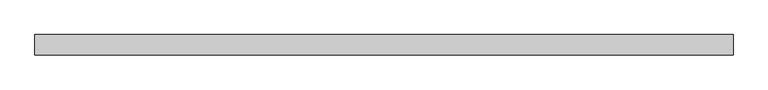
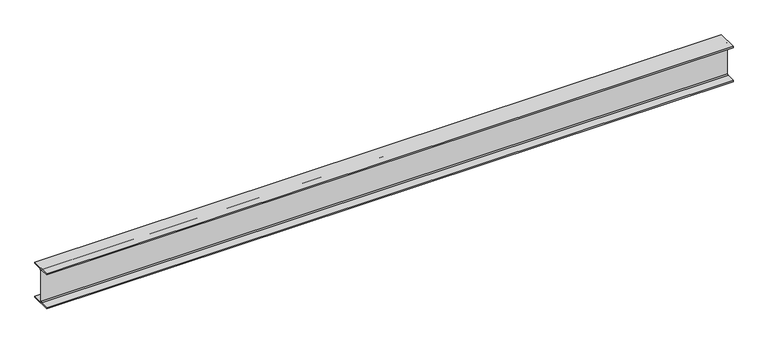
"""IFC4 building model written with IfcOpenShell, lengths in millimetres: beam geometry, Old_Steel Beam_H-KSD3502 : H_SB_ASB_H-200×200x8x12."""

import ifcopenshell
import ifcopenshell.guid

model = None  # the IFC model being written
_history = None  # IfcOwnerHistory: only IFC2X3 demands one
_inside = {}  # id of a spatial element -> (the spatial element, [elements in it])
_under = {}  # id of a project, library or spatial element -> (it, [spatial elements below it])
_declared = {}  # id of a project -> (the project, [libraries it declares])
_typed = {}  # id of a type object -> (the type object, [elements of that type])
_made_of = {}  # id of a material, layer set ... -> (it, [elements and type objects made of it])


def new_model(schema):
    """Start an empty IFC model of exactly this schema.

    Asked for "IFC4X3", IfcOpenShell would pick the latest addendum, in which some entities
    have other attributes; the version numbers below select the first issue.
    IFC2X3 requires an IfcOwnerHistory on every rooted entity: one is made here for all.
    """
    global model, _history
    if schema == "IFC4X3":
        model = ifcopenshell.file(schema_version=(4, 3, 0, 0))
    else:
        model = ifcopenshell.file(schema=schema)
    _inside.clear()
    _under.clear()
    _declared.clear()
    _typed.clear()
    _made_of.clear()
    _history = None
    if model.schema == "IFC2X3":
        org = make("IfcOrganization", Name="unknown")
        user = make(
            "IfcPersonAndOrganization",
            ThePerson=make("IfcPerson", FamilyName="unknown"),
            TheOrganization=org,
        )
        app = make(
            "IfcApplication",
            ApplicationDeveloper=org,
            Version="unknown",
            ApplicationFullName="unknown",
            ApplicationIdentifier="unknown",
        )
        _history = make(
            "IfcOwnerHistory",
            OwningUser=user,
            OwningApplication=app,
            ChangeAction="ADDED",
            CreationDate=0,
        )
    return model


def make(cls, **values):
    """One entity of the class cls with the attributes given. An attribute that is None is left unset."""
    return model.create_entity(
        cls, **{name: value for name, value in values.items() if value is not None}
    )


def rooted(cls, **values):
    """An entity with a GlobalId (a new one), such as an element, a storey or a relation."""
    return make(cls, GlobalId=ifcopenshell.guid.new(), OwnerHistory=_history, **values)


def si_unit(unit_type, name, prefix=None):
    """IfcSIUnit, for example si_unit("LENGTHUNIT", "METRE", prefix="MILLI")."""
    return make("IfcSIUnit", UnitType=unit_type, Prefix=prefix, Name=name)


def assignment(units):
    """IfcUnitAssignment: the units of a project."""
    return None if units is None else make("IfcUnitAssignment", Units=units)


def point(xyz):
    """IfcCartesianPoint."""
    return None if xyz is None else make("IfcCartesianPoint", Coordinates=xyz)


def direction(xyz):
    """IfcDirection."""
    return None if xyz is None else make("IfcDirection", DirectionRatios=xyz)


def frame(location, z_axis=None, x_axis=None):
    """IfcAxis2Placement3D, a coordinate frame: its origin and axes. An axis left out is left unset."""
    return make(
        "IfcAxis2Placement3D",
        Location=point(location),
        Axis=direction(z_axis),
        RefDirection=direction(x_axis),
    )


def frame_2d(location, x_axis=None):
    """IfcAxis2Placement2D, a coordinate frame in the plane: its origin and x axis."""
    return make(
        "IfcAxis2Placement2D", Location=point(location), RefDirection=direction(x_axis)
    )


def origin():
    """The frame at (0, 0, 0) with its axes left unset."""
    return frame((0.0, 0.0, 0.0))


def place(relative_to, where):
    """IfcLocalPlacement: puts the frame where relative to a parent placement (None: the world)."""
    return make(
        "IfcLocalPlacement", PlacementRelTo=relative_to, RelativePlacement=where
    )


def context(
    kind, dimensions, precision=None, world=None, true_north=None, identifier=None
):
    """IfcGeometricRepresentationContext, for example the 3D "Model" context."""
    return make(
        "IfcGeometricRepresentationContext",
        ContextIdentifier=identifier,
        ContextType=kind,
        CoordinateSpaceDimension=dimensions,
        Precision=precision,
        WorldCoordinateSystem=world,
        TrueNorth=true_north,
    )


def project(units=None, contexts=None):
    """IfcProject with its units and contexts."""
    return rooted(
        "IfcProject",
        Name="project",
        RepresentationContexts=contexts,
        UnitsInContext=assignment(units),
    )


def spatial(cls, under=None, at=None, **own):
    """A site, building, storey or space (cls), placed at a placement, below another one or the project."""
    s = rooted(cls, ObjectPlacement=at, **own)
    if under is not None:
        _under.setdefault(under.id(), (under, []))[1].append(s)
    return s


def polyline(points):
    """IfcPolyline through the points."""
    return make("IfcPolyline", Points=[point(p) for p in points])


def circle_curve(where, radius):
    """IfcCircle in the frame where."""
    return make("IfcCircle", Position=where, Radius=radius)


def trimmed(basis, trim1, trim2, sense, master):
    """IfcTrimmedCurve: the piece of a basis curve between two trims."""
    return make(
        "IfcTrimmedCurve",
        BasisCurve=basis,
        Trim1=trim1,
        Trim2=trim2,
        SenseAgreement=sense,
        MasterRepresentation=master,
    )


def segment(curve, same_sense, transition):
    """IfcCompositeCurveSegment."""
    return make(
        "IfcCompositeCurveSegment",
        Transition=transition,
        SameSense=same_sense,
        ParentCurve=curve,
    )


def composite_curve(segments, self_intersect=None):
    """IfcCompositeCurve: segments joined end to end."""
    return make("IfcCompositeCurve", Segments=segments, SelfIntersect=self_intersect)


def outline(outer, holes=None, kind="AREA"):
    """IfcArbitraryClosedProfileDef: a profile drawn as a closed curve; with holes, ...WithVoids."""
    if holes is None:
        return make("IfcArbitraryClosedProfileDef", ProfileType=kind, OuterCurve=outer)
    return make(
        "IfcArbitraryProfileDefWithVoids",
        ProfileType=kind,
        OuterCurve=outer,
        InnerCurves=holes,
    )


def extrude(swept, where, along, depth):
    """IfcExtrudedAreaSolid: the profile swept, set in the frame where, extruded along a direction by depth."""
    return make(
        "IfcExtrudedAreaSolid",
        SweptArea=swept,
        Position=where,
        ExtrudedDirection=direction(along),
        Depth=depth,
    )


def shape(context_of_items, identifier, shape_type, items):
    """IfcShapeRepresentation: the items that make up one representation, for example the "Body"."""
    return make(
        "IfcShapeRepresentation",
        ContextOfItems=context_of_items,
        RepresentationIdentifier=identifier,
        RepresentationType=shape_type,
        Items=items,
    )


def source(mapping_origin, context_of_items, identifier, shape_type, items):
    """IfcRepresentationMap: a shape defined once, which mapped items show again and again."""
    return make(
        "IfcRepresentationMap",
        MappingOrigin=mapping_origin,
        MappedRepresentation=shape(context_of_items, identifier, shape_type, items),
    )


def transform(
    local_origin,
    x_axis=None,
    y_axis=None,
    z_axis=None,
    scale=None,
    scale2=None,
    scale3=None,
    uniform=True,
):
    """IfcCartesianTransformationOperator3D, or its non-uniform kind. x_axis, y_axis, z_axis: its Axis1, 2, 3."""
    if uniform:
        return make(
            "IfcCartesianTransformationOperator3D",
            Axis1=direction(x_axis),
            Axis2=direction(y_axis),
            LocalOrigin=point(local_origin),
            Scale=scale,
            Axis3=direction(z_axis),
        )
    return make(
        "IfcCartesianTransformationOperator3DnonUniform",
        Axis1=direction(x_axis),
        Axis2=direction(y_axis),
        LocalOrigin=point(local_origin),
        Scale=scale,
        Axis3=direction(z_axis),
        Scale2=scale2,
        Scale3=scale3,
    )


def mapped(mapping_source, mapping_target):
    """IfcMappedItem: shows the shape of a source again, moved by a transform."""
    return make(
        "IfcMappedItem", MappingSource=mapping_source, MappingTarget=mapping_target
    )


def made_of(thing, what):
    """Note that an element or type object is made of a material, layer set ...; save() writes the relation."""
    if what is not None:
        _made_of.setdefault(what.id(), (what, []))[1].append(thing)
    return thing


def element(
    cls,
    number,
    at=None,
    inside=None,
    cuts=None,
    type_object=None,
    material=None,
    context=None,
    identifier="Body",
    shape_type=None,
    held_by="IfcProductDefinitionShape",
    body=None,
    shapes=None,
    **own,
):
    """One element of the class cls, such as IfcWall. Its Tag is "e" and its number.

    at: its placement. inside: the storey or other place that contains it. cuts: it is an
    opening in that element (IfcRelVoidsElement). A single representation is given by context,
    identifier, shape_type and body (its items); several are given by shapes. held_by: the class
    of the entity that holds the representations. save() writes the other relations.
    """
    e = rooted(cls, Tag="e%d" % number, ObjectPlacement=at, **own)
    if body is not None:
        shapes = [shape(context, identifier, shape_type, body)]
    if shapes is not None:
        e.Representation = make(held_by, Representations=shapes)
    if inside is not None:
        _inside.setdefault(inside.id(), (inside, []))[1].append(e)
    if cuts is not None:
        rooted(
            "IfcRelVoidsElement", RelatingBuildingElement=cuts, RelatedOpeningElement=e
        )
    if type_object is not None:
        _typed.setdefault(type_object.id(), (type_object, []))[1].append(e)
    return made_of(e, material)


def aggregate(whole, parts):
    """IfcRelAggregates: a whole, such as a stair, and the parts it consists of."""
    return rooted("IfcRelAggregates", RelatingObject=whole, RelatedObjects=parts)


def save(model, path):
    """Write the relations noted so far, then the file.

    IfcRelAggregates (storeys below a building ...), IfcRelContainedInSpatialStructure (elements
    in a storey), IfcRelDefinesByType, IfcRelAssociatesMaterial and IfcRelDeclares: one each for
    every whole, place, type object, material and project.
    """
    for whole, parts in _under.values():
        aggregate(whole, parts)
    for where, things in _inside.values():
        rooted(
            "IfcRelContainedInSpatialStructure",
            RelatedElements=things,
            RelatingStructure=where,
        )
    for kind, things in _typed.values():
        rooted("IfcRelDefinesByType", RelatedObjects=things, RelatingType=kind)
    for what, things in _made_of.values():
        rooted("IfcRelAssociatesMaterial", RelatedObjects=things, RelatingMaterial=what)
    for by, libraries in _declared.values():
        rooted("IfcRelDeclares", RelatingContext=by, RelatedDefinitions=libraries)
    model.write(path)


def beam_c67ea157(model_context):
    return source(origin(), model_context, "Body", "SweptSolid", [
        extrude(outline(composite_curve([segment(polyline([(82.5, -141.5), (82.5, -151.7), (-82.5, -151.7), (-82.5, -141.5), (-11.9, -141.5)]), True, "CONTINUOUS"), segment(trimmed(circle_curve(frame_2d((-11.9, -132.6)), 8.9), [point((-11.9, -141.5))], [point((-3.0, -132.6))], True, "CARTESIAN"), True, "CONTINUOUS"), segment(polyline([(-3.0, -132.6), (-3.0, 132.6)]), True, "CONTINUOUS"), segment(trimmed(circle_curve(frame_2d((-11.9, 132.6)), 8.9), [point((-3.0, 132.6))], [point((-11.9, 141.5))], True, "CARTESIAN"), True, "CONTINUOUS"), segment(polyline([(-11.9, 141.5), (-82.5, 141.5), (-82.5, 151.7), (82.5, 151.7), (82.5, 141.5), (11.9, 141.5)]), True, "CONTINUOUS"), segment(trimmed(circle_curve(frame_2d((11.9, 132.6)), 8.9), [point((11.9, 141.5))], [point((3.0, 132.6))], True, "CARTESIAN"), True, "CONTINUOUS"), segment(polyline([(3.0, 132.6), (3.0, -132.6)]), True, "CONTINUOUS"), segment(trimmed(circle_curve(frame_2d((11.9, -132.6)), 8.9), [point((3.0, -132.6))], [point((11.9, -141.5))], True, "CARTESIAN"), True, "CONTINUOUS"), segment(polyline([(11.9, -141.5), (82.5, -141.5)]), True, "CONTINUOUS")], self_intersect=False)), frame((-2934.658354, 0.0, 0.0), z_axis=(1.0, 0.0, 0.0), x_axis=(0.0, 1.0, 0.0)), (0.0, 0.0, 1.0), 5622.4398071),
    ])


if __name__ == "__main__":
    model = new_model("IFC4")
    model_context = context("Model", 3, world=origin())
    ifc_project = project(units=[si_unit("LENGTHUNIT", "METRE", prefix="MILLI")], contexts=[model_context])
    site = spatial("IfcSite", under=ifc_project)
    building = spatial("IfcBuilding", under=site)
    placement = place(None, origin())
    beam_shape = beam_c67ea157(model_context)
    element("IfcBeam", 1, ObjectType="Old_Steel Beam_H-KSD3502 : H_SB_ASB_H-200×200x8x12", at=placement, inside=building, context=model_context, shape_type="MappedRepresentation", body=[
        mapped(beam_shape, transform((0.0, 0.0, 0.0), x_axis=(1.0, 0.0, 0.0), y_axis=(0.0, 1.0, 0.0), z_axis=(0.0, 0.0, 1.0))),
    ])
    save(model, "model.ifc")

# Revit data of these elements
# Type "Old_Steel Beam_H-KSD3502 : H_SB_ASB_H-200×200x8x12"
#   Width = 20.0 cm
#   Web Thickness = 0.8 cm
#   Web Fillet = 1.3 cm
#   Warping Constant = 141376.0 cm⁶
#   Torsional Moment of Inertia = 26.2485 cm⁴
#   Torsional Modulus = 1.0 cm³
#   Section Area = 63.53 cm²
#   Plastic Modulus weak axis = 244.0 cm³
#   Plastic Modulus strong axis = 525.0 cm³
#   Perimeter = 1.16 m²/m
#   Nominal Weight = 49.90 kgf/m
#   Moment of Inertia weak axis = 1600.00 cm⁴
#   Moment of Inertia strong axis = 4720.00 cm⁴
#   Height = 20.0 cm
#   Flange Thickness = 1.2 cm
#   Elastic Modulus weak axis = 160.0 cm³
#   Elastic Modulus strong axis = 472.0 cm³
#   Centroid Vertical = 10.0 cm
#   Centroid Horizontal = 10.0 cm
#   Length [instance default] = 1.5240 m
#   Structural Material [instance default] = Steel, 45-345
#   Assembly Code = ""
# Element 1 (IfcBeam, "Old_Steel Beam_H-KSD3502 : H_SB_ASB_H-200×200x8x12")
#   Structural Material = none
# Materials
#   "Steel, 45-345": class "Metal", colour RGB 189 187 185, transparency 0, Description = "Steel 345 MPa", Cost = 0
